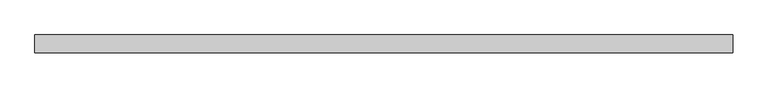
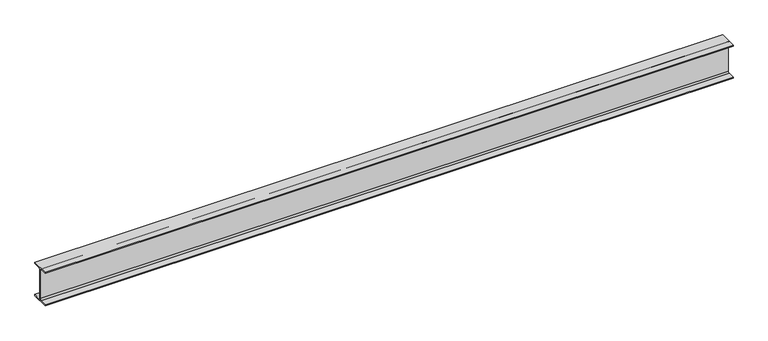
"""IFC4 building model written with IfcOpenShell, lengths in millimetres: beam geometry, 0912_Steel Framing_H-KSD3502 : H_SB_ASB_H-400x200x8x13."""

from ifc_helpers import new_model, si_unit, point, frame, frame_2d, origin, place, context, project, spatial, polyline, circle_curve, trimmed, segment, composite_curve, outline, extrude, source, transform, mapped, element, save


def beam_719eaecf(model_context):
    return source(origin(), model_context, "Body", "SweptSolid", [
        extrude(outline(composite_curve([segment(polyline([(100.0, -187.0), (100.0, -200.0), (-100.0, -200.0), (-100.0, -187.0), (-20.0, -187.0)]), True, "CONTINUOUS"), segment(trimmed(circle_curve(frame_2d((-20.0, -171.0)), 16.0), [point((-20.0, -187.0))], [point((-4.0, -171.0))], True, "CARTESIAN"), True, "CONTINUOUS"), segment(polyline([(-4.0, -171.0), (-4.0, 171.0)]), True, "CONTINUOUS"), segment(trimmed(circle_curve(frame_2d((-20.0, 171.0)), 16.0), [point((-4.0, 171.0))], [point((-20.0, 187.0))], True, "CARTESIAN"), True, "CONTINUOUS"), segment(polyline([(-20.0, 187.0), (-100.0, 187.0), (-100.0, 200.0), (100.0, 200.0), (100.0, 187.0), (20.0, 187.0)]), True, "CONTINUOUS"), segment(trimmed(circle_curve(frame_2d((20.0, 171.0)), 16.0), [point((20.0, 187.0))], [point((4.0, 171.0))], True, "CARTESIAN"), True, "CONTINUOUS"), segment(polyline([(4.0, 171.0), (4.0, -171.0)]), True, "CONTINUOUS"), segment(trimmed(circle_curve(frame_2d((20.0, -171.0)), 16.0), [point((4.0, -171.0))], [point((20.0, -187.0))], True, "CARTESIAN"), True, "CONTINUOUS"), segment(polyline([(20.0, -187.0), (100.0, -187.0)]), True, "CONTINUOUS")], self_intersect=False)), frame((-3904.8, 0.0, 0.0), z_axis=(1.0, 0.0, 0.0), x_axis=(0.0, 1.0, 0.0)), (0.0, 0.0, 1.0), 7809.6),
    ])


if __name__ == "__main__":
    model = new_model("IFC4")
    model_context = context("Model", 3, world=origin())
    ifc_project = project(units=[si_unit("LENGTHUNIT", "METRE", prefix="MILLI")], contexts=[model_context])
    site = spatial("IfcSite", under=ifc_project)
    building = spatial("IfcBuilding", under=site)
    placement = place(None, origin())
    beam_shape = beam_719eaecf(model_context)
    element("IfcBeam", 1, ObjectType="0912_Steel Framing_H-KSD3502 : H_SB_ASB_H-400x200x8x13", at=placement, inside=building, context=model_context, shape_type="MappedRepresentation", body=[
        mapped(beam_shape, transform((0.0, 0.0, 0.0), x_axis=(1.0, 0.0, 0.0), y_axis=(0.0, 1.0, 0.0), z_axis=(0.0, 0.0, 1.0))),
    ])
    save(model, "model.ifc")

# Revit data of these elements
# Type "0912_Steel Framing_H-KSD3502 : H_SB_ASB_H-400x200x8x13"
#   H_WM Code_1 = "S01AA002-00001 | Main Steel Structure Fabrication Work | Shelter/Building | Medium Steel - Standard (90KG/M>Weight≥30KG/M) | Material: (   )"
#   H_WM Code_2 = "S03AA028-00001 | Main Steel Structure Erection Work | Shelter/Building | Medium Steel (90KG/M>Weight≥30KG/M) | Material: (   )"
#   H_WM Code_3 = "S01AA010-00001 | Main Steel Structure Fabrication Work | Shelter/Building | Steel Painting/Coating | for Non-Fireproofed Steel Surface, Surface Preparation, Primer, Second & Final Coat | Material: (   )"
#   H_Q'ty Cal Type Tag = "SB-Q2"
#   Width = 20.0 cm
#   Web Thickness = 0.8 cm
#   Web Fillet = 1.6 cm
#   Warping Constant = 649000.0 cm⁶
#   W = 0
#   Torsional Moment of Inertia = 35.8981 cm⁴
#   Section Area = 84.12 cm²
#   Plastic Modulus weak axis = 268.0 cm³
#   Plastic Modulus strong axis = 1330.0 cm³
#   Perimeter = 1.56 m²/m
#   Nominal Weight = 66.00 kgf/m
#   Moment of Inertia weak axis = 1740.00 cm⁴
#   Moment of Inertia strong axis = 23700.00 cm⁴
#   Height = 40.0 cm
#   Flange Thickness = 1.3 cm
#   Elastic Modulus weak axis = 174.0 cm³
#   Elastic Modulus strong axis = 1190.0 cm³
#   Centroid Vertical = 20.0 cm
#   Centroid Horizontal = 10.0 cm
#   Ix = 237000000
#   Length [instance default] = 1.5240 m
#   Zx = 1330000
#   b = 0.2000 m
#   h = 0.4000 m
#   r = 0.0160 m
#   s = 0.0080 m
#   t = 0.0130 m
#   A = 0.008412 m²
#   Structural Material [instance default] = Steel, 45-345
#   Assembly Code = ""
# Element 1 (IfcBeam, "0912_Steel Framing_H-KSD3502 : H_SB_ASB_H-400x200x8x13")
#   Structural Material = none
# Materials
#   "Steel, 45-345": class "Metal", colour RGB 189 187 185, transparency 0, Description = "Steel 345 MPa", Cost = 0
